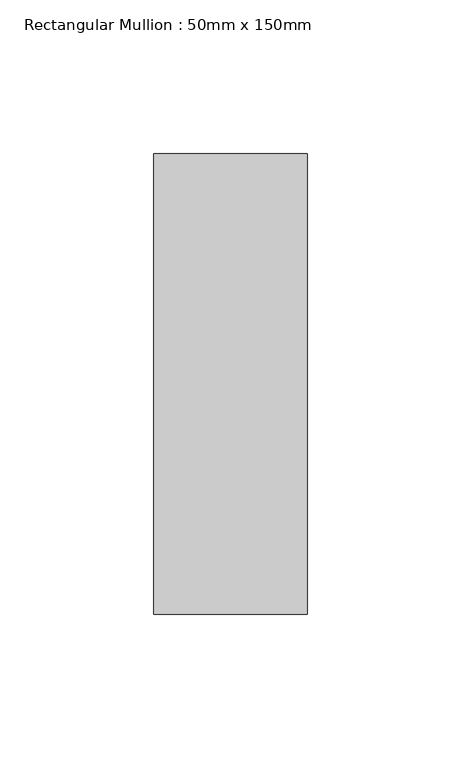
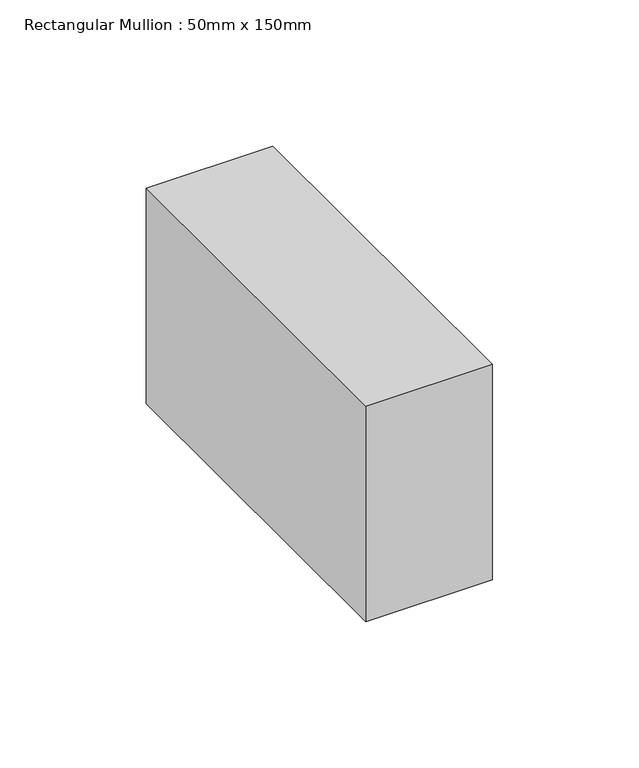
"""IFC4 building model written with IfcOpenShell, lengths in millimetres: member geometry, Rectangular Mullion : 50mm x 150mm."""

from ifc_helpers import new_model, si_unit, frame, origin, place, context, project, spatial, polyline, outline, extrude, source, transform, mapped, element, save


def rectangular_mullion_50mm_x_150mm_d3cccc3e(model_context):
    return source(origin(), model_context, "Body", "SweptSolid", [
        extrude(outline(polyline([(0.0, 75.0), (0.0, -75.0), (-50.0, -75.0), (-50.0, 75.0), (0.0, 75.0)])), frame((0.0, 0.0, -89.9999997), z_axis=(0.0, 0.0, 1.0), x_axis=(1.0, 0.0, 0.0)), (0.0, 0.0, 1.0), 89.9999997),
    ])


if __name__ == "__main__":
    model = new_model("IFC4")
    model_context = context("Model", 3, world=origin())
    ifc_project = project(units=[si_unit("LENGTHUNIT", "METRE", prefix="MILLI")], contexts=[model_context])
    site = spatial("IfcSite", under=ifc_project)
    building = spatial("IfcBuilding", under=site)
    placement = place(None, origin())
    rectangular_mullion_50mm_x_150mm_shape = rectangular_mullion_50mm_x_150mm_d3cccc3e(model_context)
    element("IfcMember", 1, ObjectType="Rectangular Mullion : 50mm x 150mm", at=placement, inside=building, context=model_context, shape_type="MappedRepresentation", body=[
        mapped(rectangular_mullion_50mm_x_150mm_shape, transform((0.0, 0.0, 0.0), x_axis=(1.0, 0.0, 0.0), y_axis=(0.0, 1.0, 0.0), z_axis=(0.0, 0.0, 1.0))),
    ])
    save(model, "model.ifc")

# Revit data of these elements
# Type "Rectangular Mullion : 50mm x 150mm"
#   built-in parameter 1007304 = 0.492126 (stored number, unit not read)
#   built-in parameter 1007301 = 0.082021 (stored number, unit not read)
#   built-in parameter 1007300 = 0.082021 (stored number, unit not read)
# Element 1 (IfcMember, "Rectangular Mullion : 50mm x 150mm")
#   Materials on its faces: "Aluminum"
# Materials
#   "Aluminum": class "Metal", colour RGB 244 244 244, transparency 0, Description = "Aluminum 6061", Cost = 0
